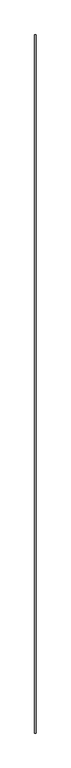
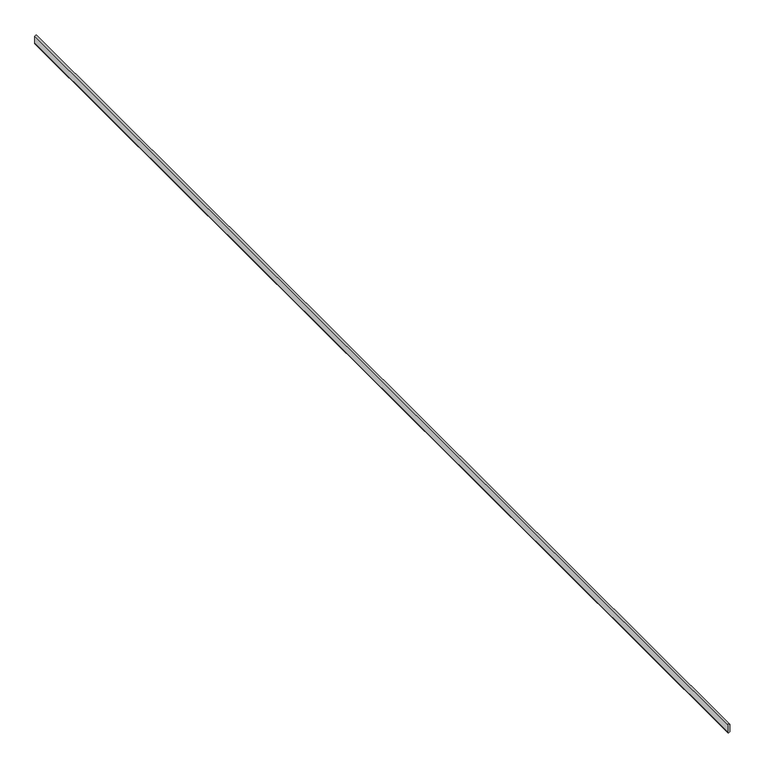
"""IFC4 building model written with IfcOpenShell, lengths in millimetres: proxy geometry, Joint038 3405 : Joint038 3405."""

from ifc_helpers import new_model, si_unit, point, frame, frame_2d, origin, place, context, project, spatial, polyline, circle_curve, trimmed, segment, composite_curve, outline, extrude, source, transform, mapped, element, save


def generic_models_dcd0c69b(model_context):
    return source(origin(), model_context, "Body", "SweptSolid", [
        extrude(outline(composite_curve([segment(trimmed(circle_curve(frame_2d((43051.539923, 17735.4480606)), 1.765625), [point((43051.539923, 17737.2136856))], [point((43051.539923, 17733.6824356))], False, "CARTESIAN"), True, "CONTINUOUS"), segment(polyline([(43051.539923, 17733.6824356), (43039.465216, 17733.6824356)]), True, "CONTINUOUS"), segment(trimmed(circle_curve(frame_2d((43039.465216, 17735.4480606)), 1.765625), [point((43039.465216, 17733.6824356))], [point((43039.465216, 17737.2136856))], False, "CARTESIAN"), True, "CONTINUOUS"), segment(polyline([(43039.465216, 17737.2136856), (43051.539923, 17737.2136856)]), True, "CONTINUOUS")], self_intersect=False)), frame((0.0, 7982.1507711, 0.0), z_axis=(0.0, 1.0, 0.0), x_axis=(0.0, 0.0, 1.0)), (0.0, 0.0, 1.0), 2000.0),
    ])


if __name__ == "__main__":
    model = new_model("IFC4")
    model_context = context("Model", 3, world=origin())
    ifc_project = project(units=[si_unit("LENGTHUNIT", "METRE", prefix="MILLI")], contexts=[model_context])
    site = spatial("IfcSite", under=ifc_project)
    building = spatial("IfcBuilding", under=site)
    placement = place(None, origin())
    generic_models_shape = generic_models_dcd0c69b(model_context)
    element("IfcBuildingElementProxy", 1, Name="Joint038 3405 : Joint038 3405", ObjectType="Joint038 3405 : Joint038 3405", at=placement, inside=building, context=model_context, shape_type="MappedRepresentation", body=[
        mapped(generic_models_shape, transform((0.0, 0.0, 0.0), x_axis=(1.0, 0.0, 0.0), y_axis=(0.0, 1.0, 0.0), z_axis=(0.0, 0.0, 1.0))),
    ])
    save(model, "model.ifc")

# Revit data of these elements
# Type "Joint038 3405 : Joint038 3405"
#   NameOverride = "Joint038"
# Element 1 (IfcBuildingElementProxy, "Joint038 3405 : Joint038 3405")
#   Materials on its faces: "SEALANT"
# Materials
#   "SEALANT": class "Unassigned", colour RGB 142 225 148, transparency 0
